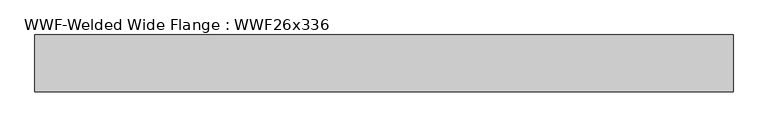
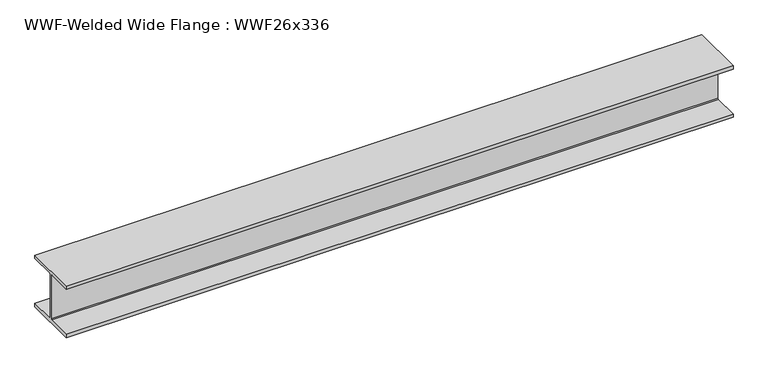
"""IFC4 building model written with IfcOpenShell, lengths in millimetres: beam geometry, WWF-Welded Wide Flange : WWF26x336."""

from ifc_helpers import new_model, si_unit, frame, origin, place, context, project, spatial, polyline, outline, extrude, source, transform, mapped, element, save


def wwf_welded_wide_flange_wwf26x336_dcec3f82(model_context):
    return source(origin(), model_context, "Body", "SweptSolid", [
        extrude(outline(polyline([(324.993, -284.988), (324.993, -324.993), (-324.993, -324.993), (-324.993, -284.988), (-20.6375, -284.988), (-9.9949, -274.3454), (-9.9949, 274.3454), (-20.6375, 284.988), (-324.993, 284.988), (-324.993, 324.993), (324.993, 324.993), (324.993, 284.988), (20.6375, 284.988), (9.9949, 274.3454), (9.9949, -274.3454), (20.6375, -284.988), (324.993, -284.988)])), frame((-3934.8877112, 0.0, 0.0), z_axis=(1.0, 0.0, 0.0), x_axis=(0.0, 1.0, 0.0)), (0.0, 0.0, 1.0), 7999.1210166),
    ])


if __name__ == "__main__":
    model = new_model("IFC4")
    model_context = context("Model", 3, world=origin())
    ifc_project = project(units=[si_unit("LENGTHUNIT", "METRE", prefix="MILLI")], contexts=[model_context])
    site = spatial("IfcSite", under=ifc_project)
    building = spatial("IfcBuilding", under=site)
    placement = place(None, origin())
    wwf_welded_wide_flange_wwf26x336_shape = wwf_welded_wide_flange_wwf26x336_dcec3f82(model_context)
    element("IfcBeam", 1, ObjectType="WWF-Welded Wide Flange : WWF26x336", at=placement, inside=building, context=model_context, shape_type="MappedRepresentation", body=[
        mapped(wwf_welded_wide_flange_wwf26x336_shape, transform((0.0, 0.0, 0.0), x_axis=(1.0, 0.0, 0.0), y_axis=(0.0, 1.0, 0.0), z_axis=(0.0, 0.0, 1.0))),
    ])
    save(model, "model.ifc")

# Revit data of these elements
# Type "WWF-Welded Wide Flange : WWF26x336"
#   Assembly Code = "B10"
#   Nominal d = "12"
#   W = 336
#   Length [instance default] = 1524 mm
#   bf = 649.986 mm
#   d = 649.986 mm
#   k = 20.638 mm
#   tf = 40.005 mm
#   tw = 19.99 mm
#   A = 0.0635483 m²
#   Structural Material [instance default] = Steel ASTM A572
# Element 1 (IfcBeam, "WWF-Welded Wide Flange : WWF26x336")
#   Structural Material = Metal - Steel 43-275
#   Materials on its faces: "Metal - Steel 43-275"
# Materials
#   "Steel ASTM A572": class "Metal", colour RGB 247 247 247, transparency 0, Description = "Structural steel, high strength low alloy, ASTM - A572 - 50", Cost = 0
#   "Metal - Steel 43-275": class "Metal", colour RGB 247 247 247, transparency 0, Cost = 0
